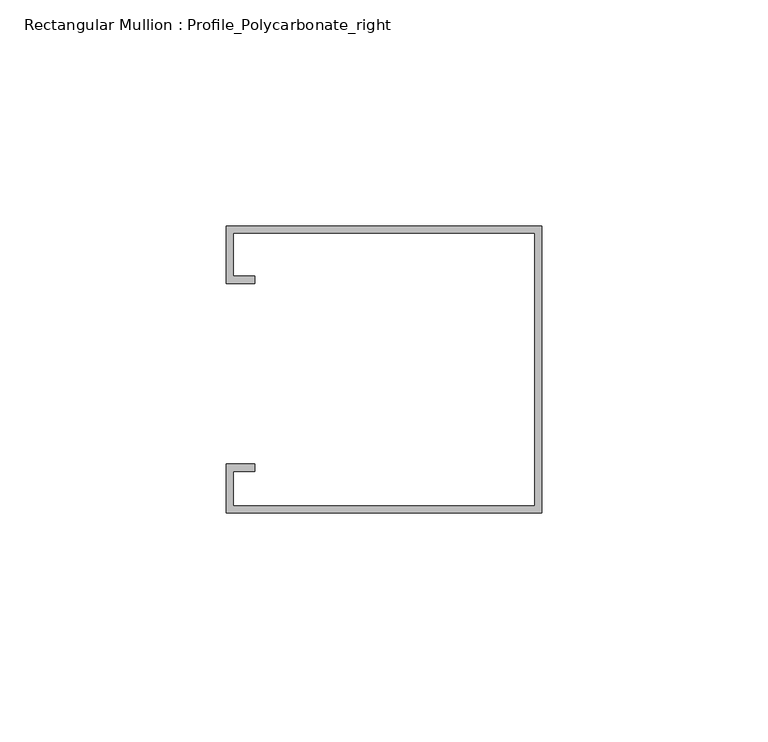
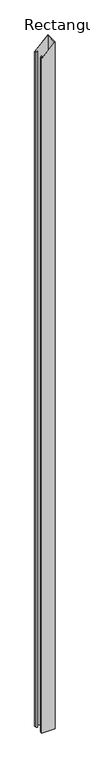
"""IFC4 building model written with IfcOpenShell, lengths in millimetres: member geometry, Rectangular Mullion : Profile_Polycarbonate_right."""

from ifc_helpers import new_model, si_unit, origin, place, context, project, spatial, faceted_brep, source, transform, mapped, element, save


def rectangular_mullion_profile_polycarbonate_right_f9876bef(model_context):
    return source(origin(), model_context, "Body", "Brep", [
        faceted_brep([(0.0, 32.7, -3772.1642939), (0.0, -30.8, -3772.1642939), (-69.85, -30.8, -3772.1642939), (-69.85, -20.0, -3772.1642939), (-63.5, -20.0, -3772.1642939), (-63.5, -21.5875, -3772.1642939), (-68.2625, -21.5875, -3772.1642939), (-68.2625, -29.2125, -3772.1642939), (-1.5875, -29.2125, -3772.1642939), (-1.5875, 31.1125, -3772.1642939), (-68.2625, 31.1125, -3772.1642939), (-68.2625, 21.5875, -3772.1642939), (-63.5, 21.5875, -3772.1642939), (-63.5, 20.0, -3772.1642939), (-69.85, 20.0, -3772.1642939), (-69.85, 32.7, -3772.1642939), (-69.85, 32.7, -67.0001907), (0.0, 32.7, 0.0), (-69.85, 20.0, -67.0001907), (-63.5, 20.0, -60.9092643), (-63.5, 21.5875, -60.9092643), (-68.2625, 21.5875, -65.4774591), (-68.2625, 31.1125, -65.4774591), (-1.5875, 31.1125, -1.5227316), (-1.5875, -29.2125, -1.5227316), (-68.2625, -29.2125, -65.4774591), (-68.2625, -21.5875, -65.4774591), (-63.5, -21.5875, -60.9092643), (-63.5, -20.0, -60.9092643), (-69.85, -20.0, -67.0001907), (-69.85, -30.8, -67.0001907), (0.0, -30.8, 0.0)], [[[0, 1, 2, 3, 4, 5, 6, 7, 8, 9, 10, 11, 12, 13, 14, 15]], [[16, 17, 0, 15]], [[18, 16, 15, 14]], [[19, 18, 14, 13]], [[20, 19, 13, 12]], [[21, 20, 12, 11]], [[22, 21, 11, 10]], [[23, 22, 10, 9]], [[24, 23, 9, 8]], [[25, 24, 8, 7]], [[26, 25, 7, 6]], [[27, 26, 6, 5]], [[28, 27, 5, 4]], [[29, 28, 4, 3]], [[30, 29, 3, 2]], [[31, 30, 2, 1]], [[17, 31, 1, 0]], [[17, 16, 18, 19, 20, 21, 22, 23, 24, 25, 26, 27, 28, 29, 30, 31]]]),
    ])


if __name__ == "__main__":
    model = new_model("IFC4")
    model_context = context("Model", 3, world=origin())
    ifc_project = project(units=[si_unit("LENGTHUNIT", "METRE", prefix="MILLI")], contexts=[model_context])
    site = spatial("IfcSite", under=ifc_project)
    building = spatial("IfcBuilding", under=site)
    placement = place(None, origin())
    rectangular_mullion_profile_polycarbonate_right_shape = rectangular_mullion_profile_polycarbonate_right_f9876bef(model_context)
    element("IfcMember", 1, ObjectType="Rectangular Mullion : Profile_Polycarbonate_right", at=placement, inside=building, context=model_context, shape_type="MappedRepresentation", body=[
        mapped(rectangular_mullion_profile_polycarbonate_right_shape, transform((0.0, 0.0, 0.0), x_axis=(1.0, 0.0, 0.0), y_axis=(0.0, 1.0, 0.0), z_axis=(0.0, 0.0, 1.0))),
    ])
    save(model, "model.ifc")

# Revit data of these elements
# Type "Rectangular Mullion : Profile_Polycarbonate_right"
#   built-in parameter 1007322 = 0.208333 (stored number, unit not read)
#   built-in parameter 1007321 = 0 (stored number, unit not read)
#   built-in parameter 1007320 = 0.00520833 (stored number, unit not read)
